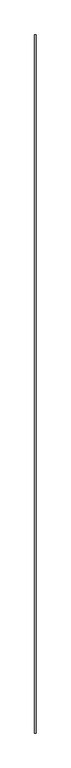
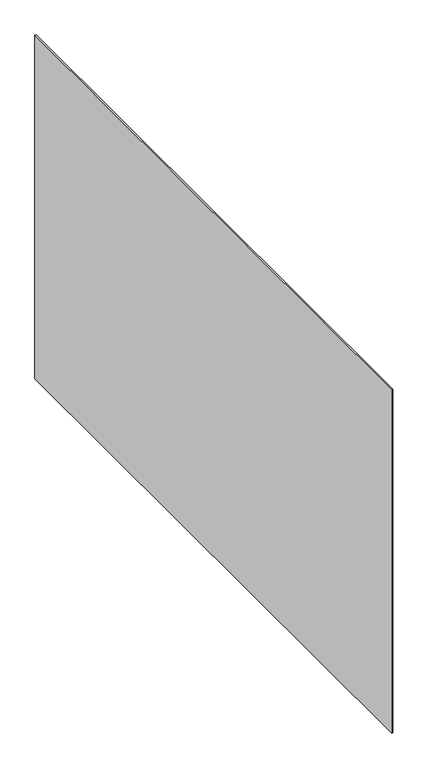
"""IFC4 building model written with IfcOpenShell, lengths in millimetres: proxy geometry, Generic Models 7:Generic Models 1:5:Generic Models 1:5 : Generic Models 7:Generic Models 1:337419:34 : Generic Models 7:Generic Models 1:5:Generic Models 1:5 : Generic Models 7:Generic Models 1:337419:311462."""

from ifc_helpers import new_model, si_unit, frame, origin, place, context, project, spatial, polyline, outline, extrude, source, transform, mapped, element, save


def generic_models_3e096008(model_context):
    return source(origin(), model_context, "Body", "SweptSolid", [
        extrude(outline(polyline([(667566.3617239, -568258.7697175), (667585.4117239, -568258.7697175), (667585.4117239, -578724.4663841), (667566.3617239, -578724.4663841), (667566.3617239, -568258.7697175)])), frame((0.0, 0.0, 6.35), z_axis=(0.0, 0.0, 1.0), x_axis=(1.0, 0.0, 0.0)), (0.0, 0.0, 1.0), 6148.740949),
    ])


if __name__ == "__main__":
    model = new_model("IFC4")
    model_context = context("Model", 3, world=origin())
    ifc_project = project(units=[si_unit("LENGTHUNIT", "METRE", prefix="MILLI")], contexts=[model_context])
    site = spatial("IfcSite", under=ifc_project)
    building = spatial("IfcBuilding", under=site)
    placement = place(None, origin())
    generic_models_shape = generic_models_3e096008(model_context)
    element("IfcBuildingElementProxy", 1, Name="Generic Models 7:Generic Models 1:5:Generic Models 1:5 : Generic Models 7:Generic Models 1:337419:34 : Generic Models 7:Generic Models 1:5:Generic Models 1:5 : Generic Models 7:Generic Models 1:337419:311462", ObjectType="Generic Models 7:Generic Models 1:5:Generic Models 1:5 : Generic Models 7:Generic Models 1:337419:34 : Generic Models 7:Generic Models 1:5:Generic Models 1:5 : Generic Models 7:Generic Models 1:337419:311462", at=placement, inside=building, context=model_context, shape_type="MappedRepresentation", body=[
        mapped(generic_models_shape, transform((0.0, 0.0, 0.0), x_axis=(1.0, 0.0, 0.0), y_axis=(0.0, 1.0, 0.0), z_axis=(0.0, 0.0, 1.0))),
    ])
    save(model, "model.ifc")

# Revit data of these elements
# Type "Generic Models 7:Generic Models 1:5:Generic Models 1:5 : Generic Models 7:Generic Models 1:337419:34 : Generic Models 7:Generic Models 1:5:Generic Models 1:5 : Generic Models 7:Generic Models 1:337419:311462"
#   NameOverride = "Generic Models 7:Generic Models 1:5:Generic Models 1:5 : Generic Models 7:Generic Models 1:337419:311462"
#   ObjectTypeOverride = "Generic Models 1:5 : Generic Models 7:Generic Models 1:337419"
#   Reference = "Generic Models 1"
#   Tag = "311462"
# Element 1 (IfcBuildingElementProxy, "Generic Models 7:Generic Models 1:5:Generic Models 1:5 : Generic Models 7:Generic Models 1:337419:34 : Generic Models 7:Generic Models 1:5:Generic Models 1:5 : Generic Models 7:Generic Models 1:337419:311462")
#   Materials on its faces: "1\" MINERAL WOOL BOARD INSULATION - BLACK MAT FACER"
# Materials
#   "1\" MINERAL WOOL BOARD INSULATION - BLACK MAT FACER": class "Unassigned", colour RGB 205 188 106, transparency 0, Cost = 0
